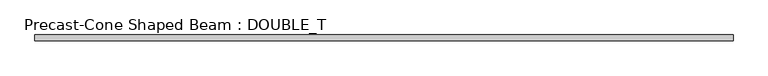
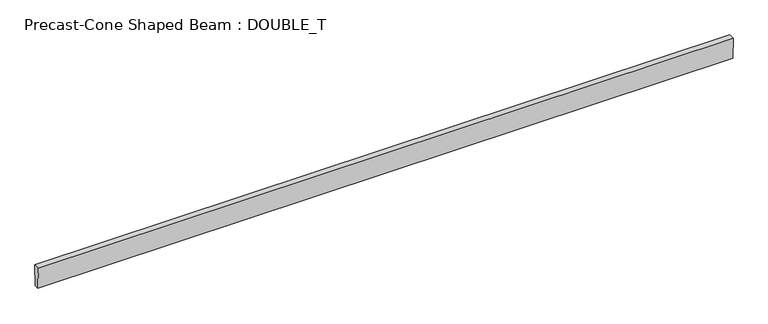
"""IFC4 building model written with IfcOpenShell, lengths in millimetres: beam geometry, Precast-Cone Shaped Beam : DOUBLE_T."""

from ifc_helpers import new_model, si_unit, frame, origin, place, context, project, spatial, polyline, outline, extrude, source, transform, mapped, element, save


def precast_cone_shaped_beam_double_t_3d71fa44(model_context):
    return source(origin(), model_context, "Body", "SweptSolid", [
        extrude(outline(polyline([(50.8, -228.6), (-50.8, -228.6), (-63.5, 228.6), (63.5, 228.6), (50.8, -228.6)])), frame((-7353.3, 0.0, 0.0), z_axis=(1.0, 0.0, 0.0), x_axis=(0.0, 1.0, 0.0)), (0.0, 0.0, 1.0), 14859.0),
    ])


if __name__ == "__main__":
    model = new_model("IFC4")
    model_context = context("Model", 3, world=origin())
    ifc_project = project(units=[si_unit("LENGTHUNIT", "METRE", prefix="MILLI")], contexts=[model_context])
    site = spatial("IfcSite", under=ifc_project)
    building = spatial("IfcBuilding", under=site)
    placement = place(None, origin())
    precast_cone_shaped_beam_double_t_shape = precast_cone_shaped_beam_double_t_3d71fa44(model_context)
    element("IfcBeam", 1, ObjectType="Precast-Cone Shaped Beam : DOUBLE_T", at=placement, inside=building, context=model_context, shape_type="MappedRepresentation", body=[
        mapped(precast_cone_shaped_beam_double_t_shape, transform((0.0, 0.0, 0.0), x_axis=(1.0, 0.0, 0.0), y_axis=(0.0, 1.0, 0.0), z_axis=(0.0, 0.0, 1.0))),
    ])
    save(model, "model.ifc")

# Revit data of these elements
# Type "Precast-Cone Shaped Beam : DOUBLE_T"
#   Top Width = 0' - 5"
#   Tie Rod Weight [instance default] = 30
#   Tie Rod W [instance default] = 0.0660938 kip
#   Single Rebar Weight [instance default] = 50
#   Single Rebar W [instance default] = 0.110156 kip
#   Rebar Grids Weight [instance default] = 100
#   Rebar Grids W [instance default] = 0.220313 kip
#   Depth = 1' - 6"
#   Bottom Width = 0' - 4"
#   Length [instance default] = 5' - 0"
#   Structural Material [instance default] = Concrete, Precast
#   Assembly Code = ""
# Element 1 (IfcBeam, "Precast-Cone Shaped Beam : DOUBLE_T")
#   Length = 49' - 3"
#   Structural Material = Concrete - Precast Concrete - Normal Weight Concrete - 5 ksi
#   Materials on its faces: "Concrete - Precast Concrete - Normal Weight Concrete - 5 ksi"
# Materials
#   "Concrete, Precast": class "Concrete", colour RGB 198 187 187, transparency 0, Description = "Precast concrete", Cost = 0
#   "Concrete - Precast Concrete - Normal Weight Concrete - 5 ksi": class "Concrete", colour RGB 198 187 187, transparency 0, Cost = 0
